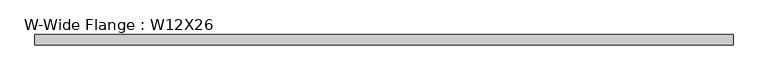
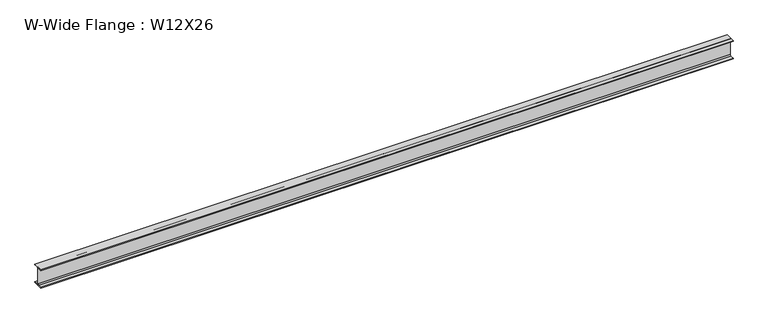
"""IFC4 building model written with IfcOpenShell, lengths in millimetres: beam geometry, W-Wide Flange : W12X26."""

from ifc_helpers import new_model, si_unit, point, frame, frame_2d, origin, place, context, project, spatial, polyline, circle_curve, trimmed, segment, composite_curve, outline, extrude, source, transform, mapped, element, save


def w_wide_flange_w12x26_16ae085f(model_context):
    return source(origin(), model_context, "Body", "SweptSolid", [
        extrude(outline(composite_curve([segment(polyline([(82.4011719, -145.5539063), (82.4011719, -155.178125), (-82.4011719, -155.178125), (-82.4011719, -145.5539063), (-20.2902344, -145.5539063)]), True, "CONTINUOUS"), segment(trimmed(circle_curve(frame_2d((-20.2902344, -128.190625)), 17.3632812), [point((-20.2902344, -145.5539063))], [point((-2.9269531, -128.190625))], True, "CARTESIAN"), True, "CONTINUOUS"), segment(polyline([(-2.9269531, -128.190625), (-2.9269531, 128.190625)]), True, "CONTINUOUS"), segment(trimmed(circle_curve(frame_2d((-20.2902344, 128.190625)), 17.3632812), [point((-2.9269531, 128.190625))], [point((-20.2902344, 145.5539062))], True, "CARTESIAN"), True, "CONTINUOUS"), segment(polyline([(-20.2902344, 145.5539062), (-82.4011719, 145.5539062), (-82.4011719, 155.178125), (82.4011719, 155.178125), (82.4011719, 145.5539062), (20.2902344, 145.5539062)]), True, "CONTINUOUS"), segment(trimmed(circle_curve(frame_2d((20.2902344, 128.190625)), 17.3632812), [point((20.2902344, 145.5539062))], [point((2.9269531, 128.190625))], True, "CARTESIAN"), True, "CONTINUOUS"), segment(polyline([(2.9269531, 128.190625), (2.9269531, -128.190625)]), True, "CONTINUOUS"), segment(trimmed(circle_curve(frame_2d((20.2902344, -128.190625)), 17.3632812), [point((2.9269531, -128.190625))], [point((20.2902344, -145.5539063))], True, "CARTESIAN"), True, "CONTINUOUS"), segment(polyline([(20.2902344, -145.5539063), (82.4011719, -145.5539063)]), True, "CONTINUOUS")], self_intersect=False)), frame((-5629.6972349, 0.0, 0.0), z_axis=(1.0, 0.0, 0.0), x_axis=(0.0, 1.0, 0.0)), (0.0, 0.0, 1.0), 11259.3944699),
    ])


if __name__ == "__main__":
    model = new_model("IFC4")
    model_context = context("Model", 3, world=origin())
    ifc_project = project(units=[si_unit("LENGTHUNIT", "METRE", prefix="MILLI")], contexts=[model_context])
    site = spatial("IfcSite", under=ifc_project)
    building = spatial("IfcBuilding", under=site)
    placement = place(None, origin())
    w_wide_flange_w12x26_shape = w_wide_flange_w12x26_16ae085f(model_context)
    element("IfcBeam", 1, ObjectType="W-Wide Flange : W12X26", at=placement, inside=building, context=model_context, shape_type="MappedRepresentation", body=[
        mapped(w_wide_flange_w12x26_shape, transform((0.0, 0.0, 0.0), x_axis=(1.0, 0.0, 0.0), y_axis=(0.0, 1.0, 0.0), z_axis=(0.0, 0.0, 1.0))),
    ])
    save(model, "model.ifc")

# Revit data of these elements
# Type "W-Wide Flange : W12X26"
#   Assembly Code = "B10"
#   W = 26
#   Length [instance default] = 5' - 0"
#   bf = 0' - 6 125/256"
#   d = 1' - 0 7/32"
#   k = 0' - 1 1/16"
#   k2 = 0' - 0 175/256"
#   tf = 0' - 0 97/256"
#   tw = 0' - 0 59/256"
#   A = 0.053125 SF
#   Structural Material [instance default] = none
# Element 1 (IfcBeam, "W-Wide Flange : W12X26")
#   Structural Material = Dark metal
#   Materials on its faces: "Dark metal"
# Materials
#   "Dark metal": class "Generic", colour RGB 44 29 29, transparency 0, Cost = 0
